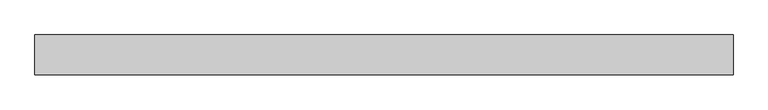
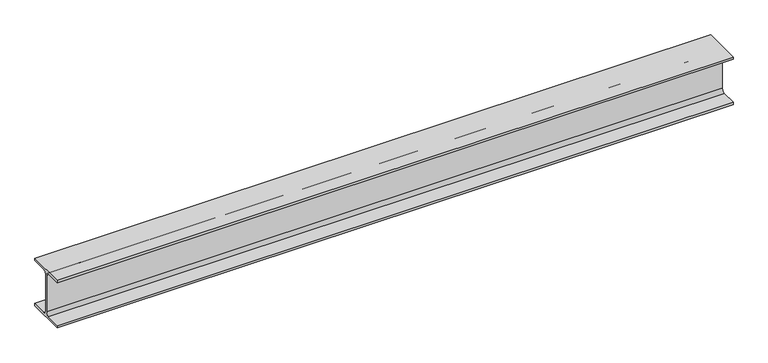
"""IFC4 building model written with IfcOpenShell, lengths in millimetres: beam geometry, 0912_Steel Framing_H-KSD3502 : H_SB_ASB_H-194x150x6x9."""

from ifc_helpers import new_model, si_unit, point, frame, frame_2d, origin, place, context, project, spatial, polyline, circle_curve, trimmed, segment, composite_curve, outline, extrude, source, transform, mapped, element, save


def beam_4f038161(model_context):
    return source(origin(), model_context, "Body", "SweptSolid", [
        extrude(outline(composite_curve([segment(polyline([(-75.0, -88.0), (-16.0, -88.0)]), True, "CONTINUOUS"), segment(trimmed(circle_curve(frame_2d((-16.0, -75.0)), 13.0), [point((-16.0, -88.0))], [point((-3.0, -75.0))], True, "CARTESIAN"), True, "CONTINUOUS"), segment(polyline([(-3.0, -75.0), (-3.0, 75.0)]), True, "CONTINUOUS"), segment(trimmed(circle_curve(frame_2d((-16.0, 75.0)), 13.0), [point((-3.0, 75.0))], [point((-16.0, 88.0))], True, "CARTESIAN"), True, "CONTINUOUS"), segment(polyline([(-16.0, 88.0), (-75.0, 88.0), (-75.0, 97.0), (75.0, 97.0), (75.0, 88.0), (16.0, 88.0)]), True, "CONTINUOUS"), segment(trimmed(circle_curve(frame_2d((16.0, 75.0)), 13.0), [point((16.0, 88.0))], [point((3.0, 75.0))], True, "CARTESIAN"), True, "CONTINUOUS"), segment(polyline([(3.0, 75.0), (3.0, -75.0)]), True, "CONTINUOUS"), segment(trimmed(circle_curve(frame_2d((16.0, -75.0)), 13.0), [point((3.0, -75.0))], [point((16.0, -88.0))], True, "CARTESIAN"), True, "CONTINUOUS"), segment(polyline([(16.0, -88.0), (75.0, -88.0), (75.0, -97.0), (-75.0, -97.0), (-75.0, -88.0)]), True, "CONTINUOUS")], self_intersect=False)), frame((-1068.0314701, 0.0, 0.0), z_axis=(1.0, 0.0, 0.0), x_axis=(0.0, 1.0, 0.0)), (0.0, 0.0, 1.0), 2617.0588612),
    ])


if __name__ == "__main__":
    model = new_model("IFC4")
    model_context = context("Model", 3, world=origin())
    ifc_project = project(units=[si_unit("LENGTHUNIT", "METRE", prefix="MILLI")], contexts=[model_context])
    site = spatial("IfcSite", under=ifc_project)
    building = spatial("IfcBuilding", under=site)
    placement = place(None, origin())
    beam_shape = beam_4f038161(model_context)
    element("IfcBeam", 1, ObjectType="0912_Steel Framing_H-KSD3502 : H_SB_ASB_H-194x150x6x9", at=placement, inside=building, context=model_context, shape_type="MappedRepresentation", body=[
        mapped(beam_shape, transform((0.0, 0.0, 0.0), x_axis=(1.0, 0.0, 0.0), y_axis=(0.0, 1.0, 0.0), z_axis=(0.0, 0.0, 1.0))),
    ])
    save(model, "model.ifc")

# Revit data of these elements
# Type "0912_Steel Framing_H-KSD3502 : H_SB_ASB_H-194x150x6x9"
#   H_WM Code_1 = "S01AA002-00001 | Main Steel Structure Fabrication Work | Shelter/Building | Medium Steel - Standard (90KG/M>Weight≥30KG/M) | Material: (   )"
#   H_WM Code_2 = "S03AA028-00001 | Main Steel Structure Erection Work | Shelter/Building | Medium Steel (90KG/M>Weight≥30KG/M) | Material: (   )"
#   H_WM Code_3 = "S01AA010-00001 | Main Steel Structure Fabrication Work | Shelter/Building | Steel Painting/Coating | for Non-Fireproofed Steel Surface, Surface Preparation, Primer, Second & Final Coat | Material: (   )"
#   H_Q'ty Cal Type Tag = "SB-Q2"
#   Width = 15.0 cm
#   Web Thickness = 0.6 cm
#   Web Fillet = 1.3 cm
#   Warping Constant = 43316.0 cm⁶
#   W = 0
#   Torsional Moment of Inertia = 8.622 cm⁴
#   Section Area = 39.01 cm²
#   Plastic Modulus weak axis = 104.0 cm³
#   Plastic Modulus strong axis = 309.0 cm³
#   Perimeter = 0.95 m²/m
#   Nominal Weight = 30.60 kgf/m
#   Moment of Inertia weak axis = 507.00 cm⁴
#   Moment of Inertia strong axis = 2690.00 cm⁴
#   Height = 19.4 cm
#   Flange Thickness = 0.9 cm
#   Elastic Modulus weak axis = 67.6 cm³
#   Elastic Modulus strong axis = 277.0 cm³
#   Centroid Vertical = 9.7 cm
#   Centroid Horizontal = 7.5 cm
#   Ix = 26900000
#   Length [instance default] = 1.5240 m
#   Zx = 309000
#   b = 0.1500 m
#   h = 0.1940 m
#   r = 0.0130 m
#   s = 0.0060 m
#   t = 0.0090 m
#   A = 0.003901 m²
#   Structural Material [instance default] = Steel, 45-345
#   Assembly Code = ""
# Element 1 (IfcBeam, "0912_Steel Framing_H-KSD3502 : H_SB_ASB_H-194x150x6x9")
#   Structural Material = none
# Materials
#   "Steel, 45-345": class "Metal", colour RGB 189 187 185, transparency 0, Description = "Steel 345 MPa", Cost = 0
